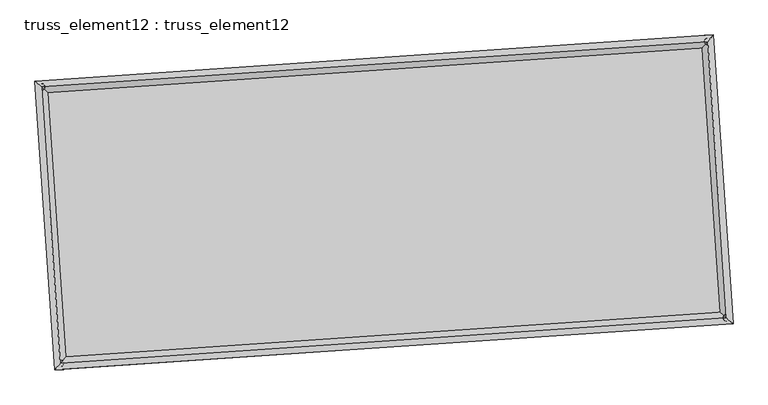
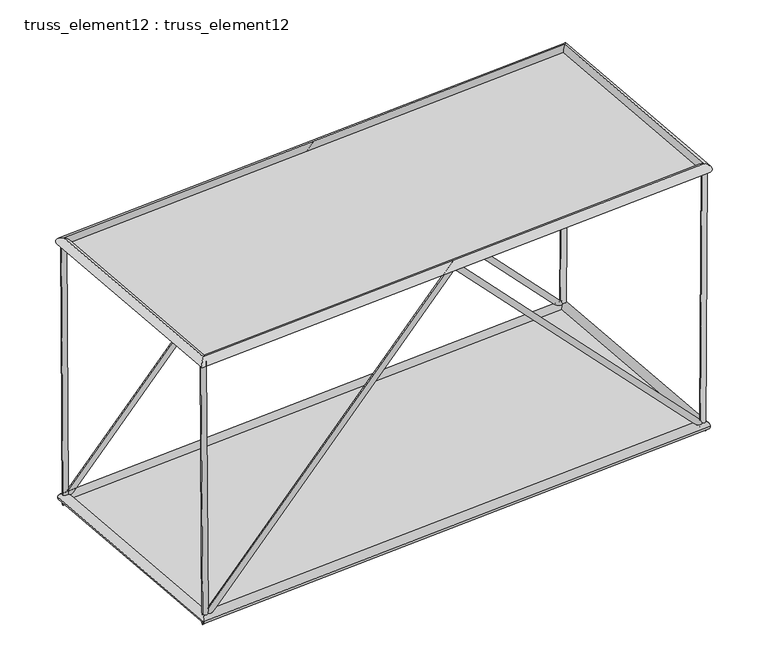
"""IFC4 building model written with IfcOpenShell, lengths in millimetres: plate geometry, truss_element12 : truss_element12."""

from ifc_helpers import new_model, si_unit, frame, origin, origin_with_axes, place, context, project, spatial, polyline, circle_curve, ellipse_curve, outline, extrude, source, transform, mapped, element, save
from ifc_brep_helpers import plane_surface, cylinder_surface, advanced_brep


def truss_element12_truss_element12_7878418a(model_context):
    return source(origin(), model_context, "Body", "SolidModel", [
        advanced_brep(
        [(-3697.7330559, 2273.9880634, 5000.2199286), (-3796.8342671, 2260.6269358, 4999.5640296), (-3665.7497354, 2276.1688844, 123.3649597), (-3763.2371475, 2262.9177957, -123.3649597), (1063.4710215, 2598.6364704, 5072.016746), (1063.9229343, 2592.0634919, 4927.7704366), (5793.1764667, 2921.1371054, 123.3684641), (5891.5845103, 2921.2433831, -123.3684641), (5824.6787759, 2923.2851281, 5000.2182213), (5924.6764587, 2923.4997973, 4999.5721856)],
        [
            (0, 1, circle_curve(frame((-3747.2836615, 2267.3074996, 4999.8919791), z_axis=(-0.0065580440171227215, -0.0004471680920716447, 0.9999783958163132), x_axis=(-0.13361132201156306, 0.9910337164155191, -0.0004330796311214912)), 50.0)),
            (1, 0, circle_curve(frame((-3747.2836615, 2267.3074996, 4999.8919791), z_axis=(-0.0065580440171227215, -0.0004471680920716447, 0.9999783958163132), x_axis=(-0.13361132201156306, 0.9910337164155191, -0.0004330796311214912)), 50.0)),
            (0, 2),
            (2, 3, ellipse_curve(frame((-3714.4934414, 2269.54334, 0.0), z_axis=(-0.9270094873495339, -0.06320925304940259, 0.36967282925972605), x_axis=(0.36881644373245154, 0.025148191295556746, 0.9291619876572165)), 133.0592395, 50.0)),
            (3, 1),
            (3, 2, ellipse_curve(frame((-3714.4934414, 2269.54334, 0.0), z_axis=(-0.9270094873495339, -0.06320925304940259, 0.36967282925972605), x_axis=(0.36881644373245154, 0.025148191295556746, 0.9291619876572165)), 133.0592395, 50.0)),
            (2, 4),
            (4, 5, ellipse_curve(frame((1063.6969779, 2595.3499811, 4999.8935913), z_axis=(-0.9976833957434984, -0.06802823820610858, -2.5773915168840048e-05), x_axis=(2.571420721554706e-05, 1.7533540442212808e-06, -0.9999999996678525)), 72.2802032, 50.0)),
            (5, 3),
            (5, 4, ellipse_curve(frame((1063.6969779, 2595.3499811, 4999.8935913), z_axis=(-0.9976833957434984, -0.06802823820610858, -2.5773915168840048e-05), x_axis=(2.571420721554706e-05, 1.7533540442212808e-06, -0.9999999996678525)), 72.2802032, 50.0)),
            (4, 6),
            (6, 7, ellipse_curve(frame((5842.3804885, 2921.1902443, 0.0), z_axis=(-0.9269817502517963, -0.06320736176214367, -0.3697426998862667), x_axis=(-0.36888615249642426, -0.025152944471190097, 0.929134186154408)), 133.0670008, 50.0)),
            (7, 5),
            (7, 6, ellipse_curve(frame((5842.3804885, 2921.1902443, 0.0), z_axis=(-0.9269817502517963, -0.06320736176214367, -0.3697426998862667), x_axis=(-0.36888615249642426, -0.025152944471190097, 0.929134186154408)), 133.0670008, 50.0)),
            (8, 9, circle_curve(frame((5874.6776173, 2923.3924627, 4999.8952035), z_axis=(0.0064594257599789005, 0.0004404436879936221, 0.9999790406944584), x_axis=(-0.002149492172002672, 0.9999975988590792, -0.00042656708586943926)), 50.0)),
            (9, 8, circle_curve(frame((5874.6776173, 2923.3924627, 4999.8952035), z_axis=(0.0064594257599789005, 0.0004404436879936221, 0.9999790406944584), x_axis=(-0.002149492172002672, 0.9999975988590792, -0.00042656708586943926)), 50.0)),
            (6, 8),
            (9, 7),
        ],
        [
            plane_surface(frame((-3747.2836615, 2317.3074946, 4999.914338), z_axis=(-0.006558044017122149, -0.0004471680920756006, 0.9999783958163133), x_axis=(0.9999784957981195, -2.932611094408344e-06, 0.0065580433614229605))),
            cylinder_surface(frame((-3747.2836615, 2267.3074996, 4999.8919791), z_axis=(-0.0065580440171227215, -0.0004471680920716447, 0.9999783958163132), x_axis=(-0.13361132201156306, 0.9910337164155191, -0.0004330796311214912)), 50.0),
            cylinder_surface(frame((-3714.4934414, 2269.54334, 0.0), z_axis=(-0.6901312584427534, -0.047057427078693426, -0.722152646382297), x_axis=(-0.02041166390988012, 0.9987523707892875, -0.045574837566446924)), 50.0),
            cylinder_surface(frame((1063.6969779, 2595.3499811, 4999.8935913), z_axis=(-0.6901683966914209, -0.047059959394698786, 0.7221169880498334), x_axis=(-0.11534684875831876, 0.9922791014168952, -0.04557729009939607)), 50.0),
            plane_surface(frame((5874.6776173, 2873.3924675, 4999.9172261), z_axis=(0.006459425759978055, 0.0004404436879920798, 0.9999790406944582), x_axis=(0.9999791376918077, -2.845072659241059e-06, -0.006459425133417806))),
            cylinder_surface(frame((5842.3804885, 2921.1902443, 0.0), z_axis=(-0.0064594257599789005, -0.0004404436879936221, -0.9999790406944584), x_axis=(-0.002149492172002672, 0.9999975988590792, -0.00042656708586943926)), 50.0),
        ],
        [
            (0, [[1, 2]]),
            (1, [[-1, 3, 4, 5]]),
            (1, [[-2, -5, 6, -3]]),
            (2, [[-4, 7, 8, 9]]),
            (2, [[-6, -9, 10, -7]]),
            (3, [[-8, 11, 12, 13]]),
            (3, [[-10, -13, 14, -11]]),
            (4, [[15, 16]]),
            (5, [[-12, 17, -16, 18]]),
            (5, [[-14, -18, -15, -17]]),
        ],
    ),
        advanced_brep(
        [(-3425.620103, -1716.7455209, 5000.2199286), (-3524.7213142, -1730.1066485, 4999.5640296), (-3393.6367824, -1714.5646999, 123.3649597), (-3491.1241946, -1727.8157886, -123.3649597), (1335.5839744, -1392.0971139, 5072.016746), (1336.0358872, -1398.6700924, 4927.7704366), (6065.2894196, -1069.5964789, 123.3684641), (6163.6974632, -1069.4902012, -123.3684641), (6096.7917288, -1067.4484562, 5000.2182213), (6196.7894116, -1067.233787, 4999.5721856)],
        [
            (0, 1, circle_curve(frame((-3475.1707086, -1723.4260847, 4999.8919791), z_axis=(-0.006558044017122952, -0.00044716809207167603, 0.9999783958163132), x_axis=(-0.1336113220115621, 0.9910337164155192, -0.0004330796311214846)), 50.0)),
            (1, 0, circle_curve(frame((-3475.1707086, -1723.4260847, 4999.8919791), z_axis=(-0.006558044017122952, -0.00044716809207167603, 0.9999783958163132), x_axis=(-0.1336113220115621, 0.9910337164155192, -0.0004330796311214846)), 50.0)),
            (0, 2),
            (2, 3, ellipse_curve(frame((-3442.3804885, -1721.1902443, 0.0), z_axis=(-0.927009487349534, -0.06320925304940223, 0.3696728292597261), x_axis=(0.3688164437324516, 0.025148191295556586, 0.9291619876572165)), 133.0592395, 50.0)),
            (3, 1),
            (3, 2, ellipse_curve(frame((-3442.3804885, -1721.1902443, 0.0), z_axis=(-0.927009487349534, -0.06320925304940223, 0.3696728292597261), x_axis=(0.3688164437324516, 0.025148191295556586, 0.9291619876572165)), 133.0592395, 50.0)),
            (2, 4),
            (4, 5, ellipse_curve(frame((1335.8099308, -1395.3836032, 4999.8935913), z_axis=(-0.9976833957434985, -0.06802823820610843, -2.5773915170605434e-05), x_axis=(2.5714207217238277e-05, 1.7533540445864214e-06, -0.9999999996678526)), 72.2802032, 50.0)),
            (5, 3),
            (5, 4, ellipse_curve(frame((1335.8099308, -1395.3836032, 4999.8935913), z_axis=(-0.9976833957434985, -0.06802823820610843, -2.5773915170605434e-05), x_axis=(2.5714207217238277e-05, 1.7533540445864214e-06, -0.9999999996678526)), 72.2802032, 50.0)),
            (4, 6),
            (6, 7, ellipse_curve(frame((6114.4934414, -1069.54334, 0.0), z_axis=(-0.9269817502517956, -0.06320736176214367, -0.3697426998862684), x_axis=(-0.3688861524964258, -0.025152944471190226, 0.9291341861544073)), 133.0670008, 50.0)),
            (7, 5),
            (7, 6, ellipse_curve(frame((6114.4934414, -1069.54334, 0.0), z_axis=(-0.9269817502517956, -0.06320736176214367, -0.3697426998862684), x_axis=(-0.3688861524964258, -0.025152944471190226, 0.9291341861544073)), 133.0670008, 50.0)),
            (8, 9, circle_curve(frame((6146.7905702, -1067.3411216, 4999.8952035), z_axis=(0.006459425759979071, 0.0004404436879936256, 0.9999790406944583), x_axis=(-0.002149492172003178, 0.9999975988590791, -0.00042656708586943915)), 50.0)),
            (9, 8, circle_curve(frame((6146.7905702, -1067.3411216, 4999.8952035), z_axis=(0.006459425759979071, 0.0004404436879936256, 0.9999790406944583), x_axis=(-0.002149492172003178, 0.9999975988590791, -0.00042656708586943915)), 50.0)),
            (6, 8),
            (9, 7),
        ],
        [
            plane_surface(frame((-3475.1707086, -1673.4260897, 4999.914338), z_axis=(-0.006558044017122149, -0.00044716809207560177, 0.9999783958163133), x_axis=(0.9999784957981195, -2.932611094408344e-06, 0.0065580433614229605))),
            cylinder_surface(frame((-3475.1707086, -1723.4260847, 4999.8919791), z_axis=(-0.0065580440171229505, -0.0004471680920716759, 0.999978395816313), x_axis=(-0.1336113220115621, 0.9910337164155192, -0.0004330796311214846)), 50.0),
            cylinder_surface(frame((-3442.3804885, -1721.1902443, 0.0), z_axis=(-0.6901312584427537, -0.04705742707869316, -0.7221526463822968), x_axis=(-0.020411663909880064, 0.9987523707892874, -0.045574837566446605)), 50.0),
            cylinder_surface(frame((1335.8099308, -1395.3836032, 4999.8935913), z_axis=(-0.6901683966914235, -0.047059959394698994, 0.7221169880498306), x_axis=(-0.1153468487583182, 0.9922791014168953, -0.045577290099395824)), 50.0),
            plane_surface(frame((6146.7905702, -1117.3411168, 4999.9172261), z_axis=(0.006459425759978055, 0.00044044368799207986, 0.9999790406944582), x_axis=(0.9999791376918077, -2.8450726587969697e-06, -0.006459425133417806))),
            cylinder_surface(frame((6114.4934414, -1069.54334, 0.0), z_axis=(-0.006459425759979071, -0.0004404436879936256, -0.9999790406944583), x_axis=(-0.002149492172003178, 0.9999975988590791, -0.00042656708586943915)), 50.0),
        ],
        [
            (0, [[1, 2]]),
            (1, [[-1, 3, 4, 5]]),
            (1, [[-2, -5, 6, -3]]),
            (2, [[-4, 7, 8, 9]]),
            (2, [[-6, -9, 10, -7]]),
            (3, [[-8, 11, 12, 13]]),
            (3, [[-10, -13, 14, -11]]),
            (4, [[15, 16]]),
            (5, [[-12, 17, -16, 18]]),
            (5, [[-14, -18, -15, -17]]),
        ],
    ),
        advanced_brep(
        [(-3475.1698571, -1723.425141, 4909.8919791), (-3475.1715601, -1723.4270284, 5089.8919791), (-3747.2846332, 2267.308319, 5089.8919791), (-3747.2826898, 2267.3066802, 4909.8919791), (5874.6784087, 2923.3934023, 5089.8952035), (5874.6768259, 2923.3915231, 4909.8952035), (6146.7914819, -1067.3419451, 5089.8952035), (6146.7896586, -1067.3402981, 4909.8952035)],
        [
            (0, 1, ellipse_curve(frame((-3475.1707086, -1723.4260847, 4999.8919791), z_axis=(-0.7535719234054182, 0.6573654662780838, -2.364078017319096e-07), x_axis=(-0.6573654662780416, -0.7535719234054551, -2.3640780134907803e-07)), 127.2792206, 90.0)),
            (1, 2),
            (2, 3, ellipse_curve(frame((-3747.2836615, 2267.3074996, 4999.8919791), z_axis=(-0.6573654662780415, -0.7535719234054551, -2.3640779880847992e-07), x_axis=(0.7535719234054182, -0.6573654662780839, 2.3640779919131162e-07)), 127.2792206, 90.0)),
            (3, 0),
            (1, 0, ellipse_curve(frame((-3475.1707086, -1723.4260847, 4999.8919791), z_axis=(-0.7535719234054182, 0.6573654662780838, -2.364078017319096e-07), x_axis=(-0.6573654662780416, -0.7535719234054551, -2.3640780134907803e-07)), 127.2792206, 90.0)),
            (3, 2, ellipse_curve(frame((-3747.2836615, 2267.3074996, 4999.8919791), z_axis=(-0.6573654662780415, -0.7535719234054551, -2.3640779880847992e-07), x_axis=(0.7535719234054182, -0.6573654662780839, 2.3640779919131162e-07)), 127.2792206, 90.0)),
            (2, 4),
            (4, 5, ellipse_curve(frame((5874.6776173, 2923.3924627, 4999.8952035), z_axis=(-0.753571923405421, 0.6573654662780805, -2.364078053169509e-07), x_axis=(-0.6573654662780386, -0.7535719234054576, -2.3640779268284074e-07)), 127.2792206, 90.0)),
            (5, 3),
            (5, 4, ellipse_curve(frame((5874.6776173, 2923.3924627, 4999.8952035), z_axis=(-0.753571923405421, 0.6573654662780805, -2.364078053169509e-07), x_axis=(-0.6573654662780386, -0.7535719234054576, -2.3640779268284074e-07)), 127.2792206, 90.0)),
            (4, 6),
            (6, 7, ellipse_curve(frame((6146.7905702, -1067.3411216, 4999.8952035), z_axis=(0.6573654662780387, 0.7535719234054576, 2.3640779522343875e-07), x_axis=(-0.7535719234054211, 0.6573654662780807, -2.364078078575489e-07)), 127.2792206, 90.0)),
            (7, 5),
            (7, 6, ellipse_curve(frame((6146.7905702, -1067.3411216, 4999.8952035), z_axis=(0.6573654662780387, 0.7535719234054576, 2.3640779522343875e-07), x_axis=(-0.7535719234054211, 0.6573654662780807, -2.364078078575489e-07)), 127.2792206, 90.0)),
            (6, 1),
            (0, 7),
        ],
        [
            cylinder_surface(frame((-3475.1707086, -1723.4260847, 4999.8919791), z_axis=(0.06802823822870056, -0.9976833960748767, 0.0), x_axis=(-0.9976833960234631, -0.06802823822519488, -1.0152132427543063e-05)), 90.0),
            cylinder_surface(frame((-3747.2836615, 2267.3074996, 4999.8919791), z_axis=(-0.9976833960748208, -0.06802823822869773, -3.3433111559642525e-07), x_axis=(-0.06802823822214815, 0.9976833960270169, -9.817801312233482e-06)), 90.0),
            cylinder_surface(frame((5874.6776173, 2923.3924627, 4999.8952035), z_axis=(-0.06802823822870865, 0.9976833960748761, 0.0), x_axis=(0.9976833960300122, 0.06802823822564956, -9.48347018771953e-06)), 90.0),
            cylinder_surface(frame((6146.7905702, -1067.3411216, 4999.8952035), z_axis=(0.997683396074821, 0.06802823822869727, 3.3433111918937347e-07), x_axis=(0.06802823822869727, -0.9976833960265705, -9.81780129795915e-06)), 90.0),
        ],
        [
            (0, [[1, 2, 3, 4]]),
            (0, [[5, -4, 6, -2]]),
            (1, [[-3, 7, 8, 9]]),
            (1, [[-6, -9, 10, -7]]),
            (2, [[-8, 11, 12, 13]]),
            (2, [[-10, -13, 14, -11]]),
            (3, [[-12, 15, -1, 16]]),
            (3, [[-14, -16, -5, -15]]),
        ],
    ),
        advanced_brep(
        [(-3358.7115243, -1625.2761972, 0.0), (-3526.0494527, -1817.1042913, 0.0), (-3810.4074885, 2353.2123043, 0.0), (-3618.5793943, 2185.8743758, 0.0), (5926.0494527, 3017.1042913, 0.0), (5758.7115243, 2825.2761972, 0.0), (6210.4074885, -1153.2123043, 0.0), (6018.5793943, -985.8743758, 0.0)],
        [
            (0, 1, ellipse_curve(frame((-3442.3804885, -1721.1902443, 0.0), z_axis=(-0.7535719234054593, 0.6573654662780792, 0.0), x_axis=(-0.6573654662780792, -0.7535719234054593, 0.0)), 127.2792206, 90.0)),
            (1, 2),
            (2, 3, ellipse_curve(frame((-3714.4934414, 2269.54334, 0.0), z_axis=(-0.6573654662780791, -0.7535719234054593, 0.0), x_axis=(0.7535719234054593, -0.6573654662780793, 0.0)), 127.2792206, 90.0)),
            (3, 0),
            (1, 0, ellipse_curve(frame((-3442.3804885, -1721.1902443, 0.0), z_axis=(-0.7535719234054593, 0.6573654662780792, 0.0), x_axis=(-0.6573654662780792, -0.7535719234054593, 0.0)), 127.2792206, 90.0)),
            (3, 2, ellipse_curve(frame((-3714.4934414, 2269.54334, 0.0), z_axis=(-0.6573654662780791, -0.7535719234054593, 0.0), x_axis=(0.7535719234054593, -0.6573654662780793, 0.0)), 127.2792206, 90.0)),
            (2, 4),
            (4, 5, ellipse_curve(frame((5842.3804885, 2921.1902443, 0.0), z_axis=(-0.7535719234054621, 0.6573654662780759, 0.0), x_axis=(-0.6573654662780762, -0.753571923405462, 0.0)), 127.2792206, 90.0)),
            (5, 3),
            (5, 4, ellipse_curve(frame((5842.3804885, 2921.1902443, 0.0), z_axis=(-0.7535719234054621, 0.6573654662780759, 0.0), x_axis=(-0.6573654662780762, -0.753571923405462, 0.0)), 127.2792206, 90.0)),
            (4, 6),
            (6, 7, ellipse_curve(frame((6114.4934414, -1069.54334, 0.0), z_axis=(0.6573654662780762, 0.7535719234054619, 0.0), x_axis=(-0.753571923405462, 0.6573654662780763, 0.0)), 127.2792206, 90.0)),
            (7, 5),
            (7, 6, ellipse_curve(frame((6114.4934414, -1069.54334, 0.0), z_axis=(0.6573654662780762, 0.7535719234054619, 0.0), x_axis=(-0.753571923405462, 0.6573654662780763, 0.0)), 127.2792206, 90.0)),
            (6, 1),
            (0, 7),
        ],
        [
            cylinder_surface(frame((-3442.3804885, -1721.1902443, 0.0), z_axis=(0.06802823822870308, -0.9976833960748764, 0.0), x_axis=(-0.9976833960748764, -0.06802823822870308, 0.0)), 90.0),
            cylinder_surface(frame((-3714.4934414, 2269.54334, 0.0), z_axis=(-0.9976833960748765, -0.06802823822870399, 0.0), x_axis=(-0.06802823822870399, 0.9976833960748765, 0.0)), 90.0),
            cylinder_surface(frame((5842.3804885, 2921.1902443, 0.0), z_axis=(-0.06802823822871121, 0.997683396074876, 0.0), x_axis=(0.997683396074876, 0.06802823822871121, 0.0)), 90.0),
            cylinder_surface(frame((6114.4934414, -1069.54334, 0.0), z_axis=(0.9976833960748765, 0.06802823822870341, 0.0), x_axis=(0.06802823822870341, -0.9976833960748765, 0.0)), 90.0),
        ],
        [
            (0, [[1, 2, 3, 4]]),
            (0, [[5, -4, 6, -2]]),
            (1, [[-3, 7, 8, 9]]),
            (1, [[-6, -9, 10, -7]]),
            (2, [[-8, 11, 12, 13]]),
            (2, [[-10, -13, 14, -11]]),
            (3, [[-12, 15, -1, 16]]),
            (3, [[-14, -16, -5, -15]]),
        ],
    ),
        extrude(outline(polyline([(-3442.3804885, -1721.1902443), (-3714.4934414, 2269.54334), (5842.3804885, 2921.1902443), (6114.4934414, -1069.54334), (-3442.3804885, -1721.1902443)])), origin_with_axes(), (0.0, 0.0, 1.0), 20.0),
        extrude(outline(polyline([(-2000.0, 4822.1516549), (2000.0, 4822.1516549), (2000.0, -4822.1516548), (-2000.0, -4822.1516548), (-2000.0, 4822.1516549)])), frame((1199.7534544, 599.983189, 4999.8935913), z_axis=(-3.33556602840147e-07, -2.2743956508971097e-08, 0.9999999999999442), x_axis=(-0.06802823822870292, 0.9976833960748765, 0.0)), (0.0, 0.0, 1.0), 20.0),
    ])


if __name__ == "__main__":
    model = new_model("IFC4")
    model_context = context("Model", 3, world=origin())
    ifc_project = project(units=[si_unit("LENGTHUNIT", "METRE", prefix="MILLI")], contexts=[model_context])
    site = spatial("IfcSite", under=ifc_project)
    building = spatial("IfcBuilding", under=site)
    placement = place(None, origin())
    truss_element12_truss_element12_shape = truss_element12_truss_element12_7878418a(model_context)
    element("IfcPlate", 1, ObjectType="truss_element12 : truss_element12", at=placement, inside=building, context=model_context, shape_type="MappedRepresentation", body=[
        mapped(truss_element12_truss_element12_shape, transform((0.0, 0.0, 0.0), x_axis=(1.0, 0.0, 0.0), y_axis=(0.0, 1.0, 0.0), z_axis=(0.0, 0.0, 1.0))),
    ])
    save(model, "model.ifc")

# Revit data of these elements
# Type "truss_element12 : truss_element12"
#   steellbar1 = 90 mm
#   steelbar2 = 50 mm
#   offset1 = 5000 mm
#   M = Default Roof
# Element 1 (IfcPlate, "truss_element12 : truss_element12")
#   Materials on its faces: "Default Roof"
# Materials
#   "Default Roof": class "Miscellaneous", colour RGB 0 127 0, transparency 0, Comments = "Rendering appearance not upgraded Rendering appearance not upgraded ", Cost = 0
